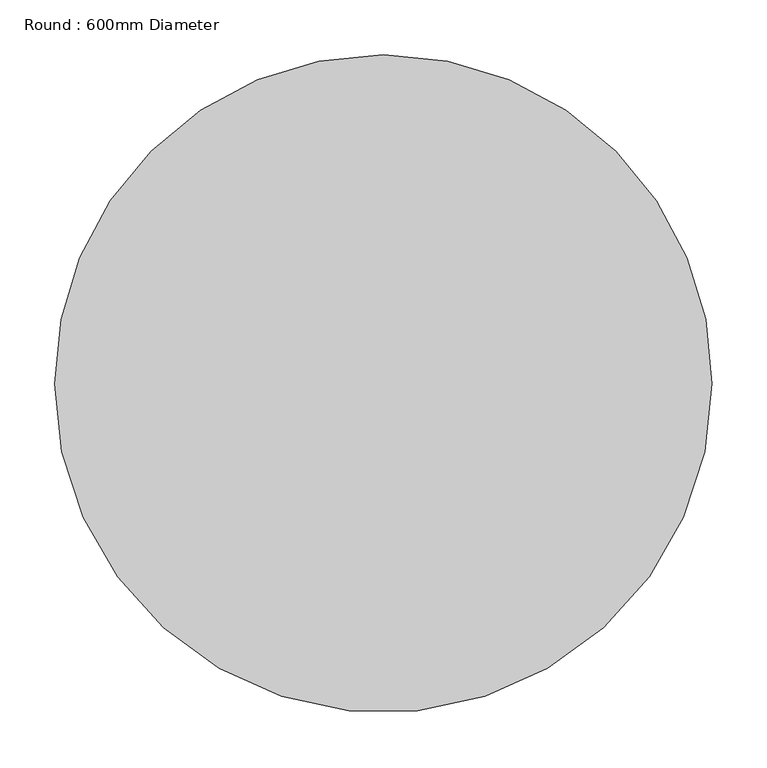
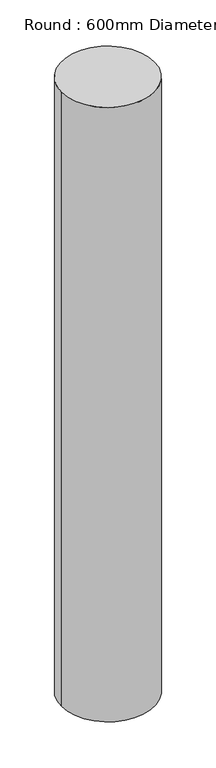
"""IFC4 building model written with IfcOpenShell, lengths in millimetres: column geometry, Round : 600mm Diameter."""

from ifc_helpers import new_model, si_unit, point, frame, origin, origin_2d, place, context, project, spatial, circle_curve, trimmed, segment, composite_curve, outline, extrude, source, transform, mapped, element, save


def round_600mm_diameter_20240e27(model_context):
    return source(origin(), model_context, "Body", "SweptSolid", [
        extrude(outline(composite_curve([segment(trimmed(circle_curve(origin_2d(), 300.0), [point((300.0, 0.0))], [point((-300.0, 0.0))], False, "CARTESIAN"), True, "CONTINUOUS"), segment(trimmed(circle_curve(origin_2d(), 300.0), [point((-300.0, 0.0))], [point((0.0, 300.0))], False, "CARTESIAN"), True, "CONTINUOUS"), segment(trimmed(circle_curve(origin_2d(), 300.0), [point((0.0, 300.0))], [point((300.0, 0.0))], False, "CARTESIAN"), True, "CONTINUOUS")], self_intersect=False)), frame((0.0, 0.0, 130470.0), z_axis=(0.0, 0.0, 1.0), x_axis=(1.0, 0.0, 0.0)), (0.0, 0.0, 1.0), 4200.0),
    ])


if __name__ == "__main__":
    model = new_model("IFC4")
    model_context = context("Model", 3, world=origin())
    ifc_project = project(units=[si_unit("LENGTHUNIT", "METRE", prefix="MILLI")], contexts=[model_context])
    site = spatial("IfcSite", under=ifc_project)
    building = spatial("IfcBuilding", under=site)
    placement = place(None, origin())
    round_600mm_diameter_shape = round_600mm_diameter_20240e27(model_context)
    element("IfcColumn", 1, ObjectType="Round : 600mm Diameter", at=placement, inside=building, context=model_context, shape_type="MappedRepresentation", body=[
        mapped(round_600mm_diameter_shape, transform((0.0, 0.0, 0.0), x_axis=(1.0, 0.0, 0.0), y_axis=(0.0, 1.0, 0.0), z_axis=(0.0, 0.0, 1.0))),
    ])
    save(model, "model.ifc")

# Revit data of these elements
# Type "Round : 600mm Diameter"
#   Keynote = "G"
#   Diameter = 600.00 mm
#   Offset Base = 0.00 mm
#   Offset Top = 0.00 mm
#   built-in parameter 1002110 = 8421504
#   built-in parameter 1002106 = element 3
#   Material = Concrete - Cast In Situ
# Element 1 (IfcColumn, "Round : 600mm Diameter")
#   Materials on its faces: "Concrete - Cast In Situ"
# Materials
#   "Concrete - Cast In Situ": class "Unassigned", colour RGB 255 255 255, transparency 0, Keynote = "E10/132", Cost = 0
